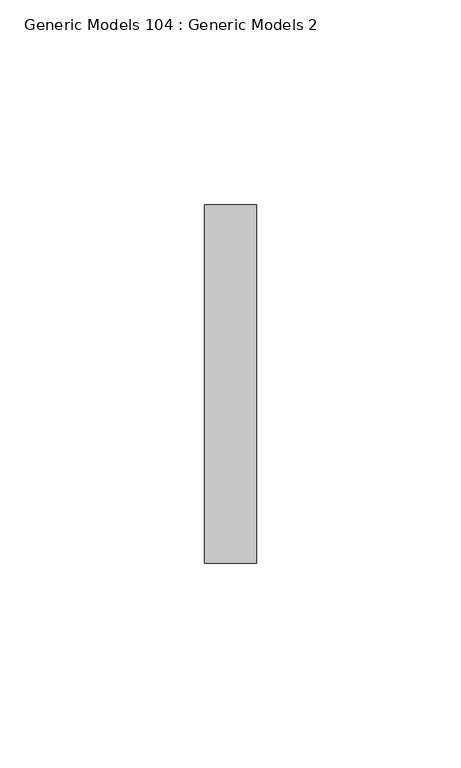
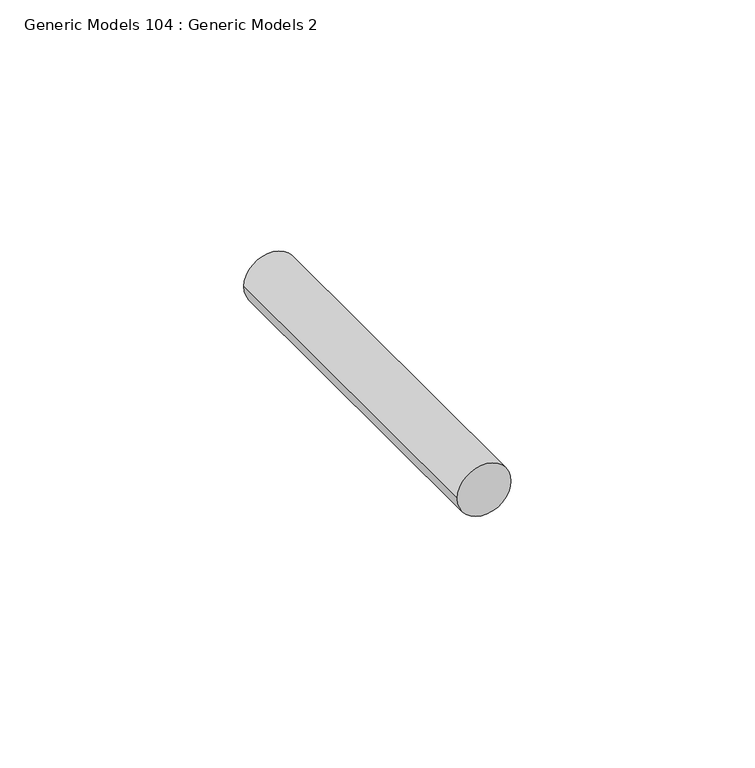
"""IFC4 building model written with IfcOpenShell, lengths in millimetres: proxy geometry, Generic Models 104 : Generic Models 2."""

from ifc_helpers import new_model, si_unit, point, frame, frame_2d, origin, place, context, project, spatial, circle_curve, trimmed, segment, composite_curve, outline, extrude, source, transform, mapped, element, save


def generic_models_104_generic_models_2_7522a2cf(model_context):
    return source(origin(), model_context, "Body", "SweptSolid", [
        extrude(outline(composite_curve([segment(trimmed(circle_curve(frame_2d((37345.8776334, 5900.5346014)), 6.35), [point((37345.8776334, 5906.8846014))], [point((37345.8776334, 5894.1846014))], False, "CARTESIAN"), True, "CONTINUOUS"), segment(trimmed(circle_curve(frame_2d((37345.8776334, 5900.5346014)), 6.35), [point((37345.8776334, 5894.1846014))], [point((37345.8776334, 5906.8846014))], False, "CARTESIAN"), True, "CONTINUOUS")], self_intersect=False)), frame((0.0, 1848.3666731, 0.0), z_axis=(0.0, 1.0, 0.0), x_axis=(0.0, 0.0, 1.0)), (0.0, 0.0, 1.0), 87.551022),
    ])


if __name__ == "__main__":
    model = new_model("IFC4")
    model_context = context("Model", 3, world=origin())
    ifc_project = project(units=[si_unit("LENGTHUNIT", "METRE", prefix="MILLI")], contexts=[model_context])
    site = spatial("IfcSite", under=ifc_project)
    building = spatial("IfcBuilding", under=site)
    placement = place(None, origin())
    generic_models_104_generic_models_2_shape = generic_models_104_generic_models_2_7522a2cf(model_context)
    element("IfcBuildingElementProxy", 1, Name="Generic Models 104 : Generic Models 2", ObjectType="Generic Models 104 : Generic Models 2", at=placement, inside=building, context=model_context, shape_type="MappedRepresentation", body=[
        mapped(generic_models_104_generic_models_2_shape, transform((0.0, 0.0, 0.0), x_axis=(1.0, 0.0, 0.0), y_axis=(0.0, 1.0, 0.0), z_axis=(0.0, 0.0, 1.0))),
    ])
    save(model, "model.ifc")

# Revit data of these elements
# Element 1 (IfcBuildingElementProxy, "Generic Models 104 : Generic Models 2")
#   Materials on its faces: "S.S. LAG BOLT - SEE STRUCT. DWGS"
# Materials
#   "S.S. LAG BOLT - SEE STRUCT. DWGS": class "Generic", colour RGB 120 120 120, transparency 0, Cost = 0
